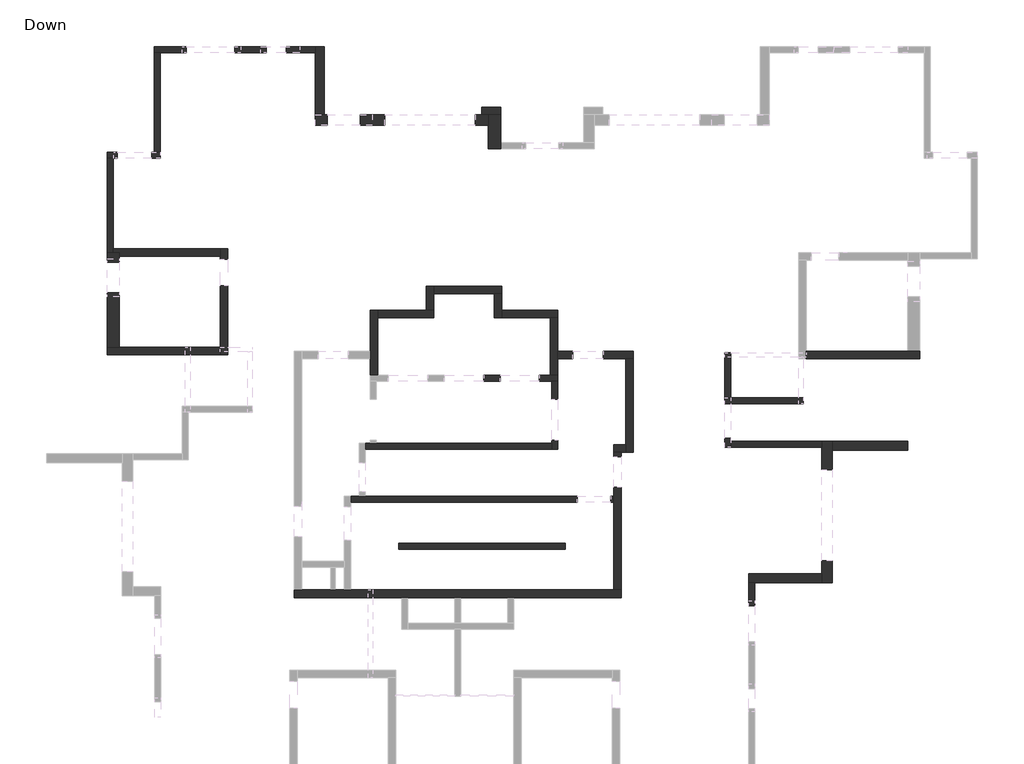
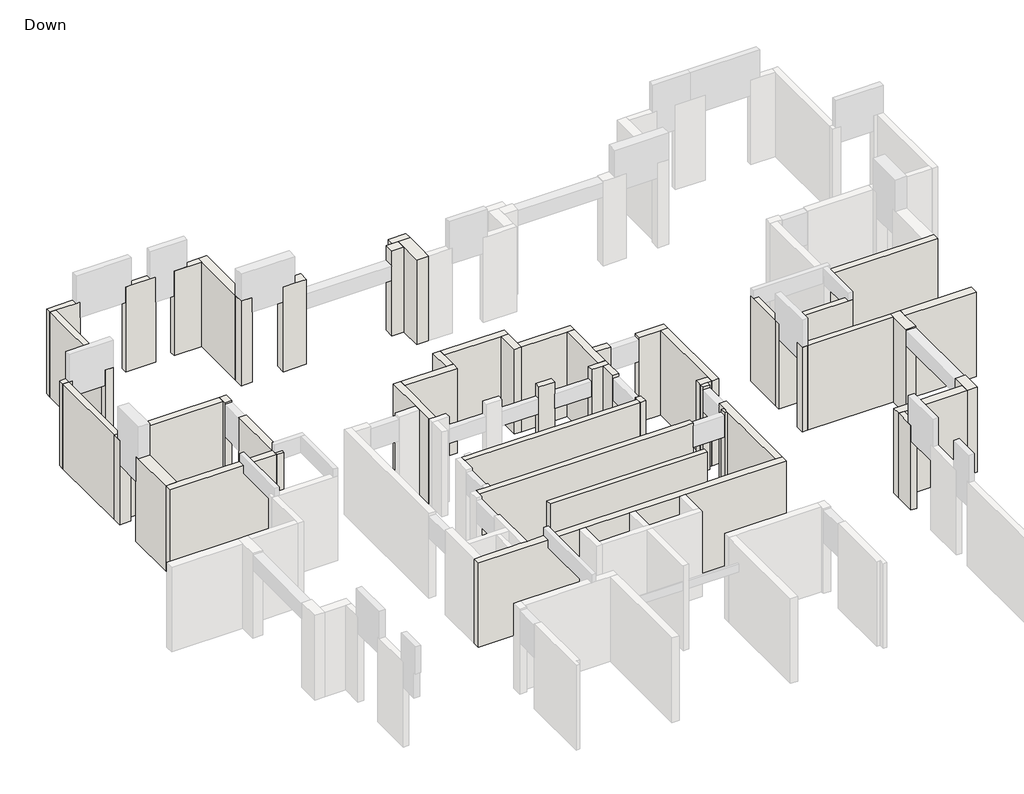
# One storey, part 2 of 3: 51 walls.
"""IFC4 building model written with IfcOpenShell, lengths in millimetres."""

from ifc_helpers import new_model, si_unit, origin, origin_with_axes, place, context, project, spatial, polyline, outline, extrude, faceted_brep, element, save

model = new_model("IFC4")

# Units and contexts
model_context = context("Model", 3, world=origin())
ifc_project = project(units=[si_unit("LENGTHUNIT", "METRE", prefix="MILLI")], contexts=[model_context])

# Site, building, storey
site = spatial("IfcSite", under=ifc_project)
building = spatial("IfcBuilding", under=site)
storey = spatial("IfcBuildingStorey", under=building, Name="Down", Elevation=0.0)

# Walls
placement = place(None, origin())
element("IfcWall", 1, ObjectType="20", at=placement, inside=storey, context=model_context, shape_type="Brep", body=[
    faceted_brep([(-24284.8686951, 10125.9195024, 0.0), (-25346.2068588, 10125.9195024, 0.0), (-25346.2068588, 10125.9195024, 3150.0), (-24424.8686951, 10125.9195024, 3150.0), (-24284.8686951, 10125.9195024, 3150.0), (-24284.8686951, 10125.9195024, 2570.0), (-24284.8686951, 9925.9195024, 0.0), (-24284.8686951, 9925.9195024, 2570.0), (-24284.8686951, 9925.9195024, 3150.0), (-24424.8686951, 9925.9195024, 3150.0), (-25146.2068588, 9925.9195024, 3150.0), (-25346.2068588, 9925.9195024, 3150.0), (-25346.2068588, 9925.9195024, 0.0), (-25146.2068588, 9925.9195024, 0.0)], [[[0, 1, 2, 3, 4, 5]], [[6, 7, 8, 9, 10, 11, 12, 13]], [[1, 0, 6, 13, 12]], [[4, 3, 2, 11, 10, 9, 8]], [[0, 5, 4, 8, 7, 6]], [[2, 1, 12, 11]]]),
])
element("IfcWall", 2, ObjectType="20", at=placement, inside=storey, context=model_context, shape_type="Brep", body=[
    faceted_brep([(-25346.2068588, 9925.9195024, 0.0), (-25346.2068588, 6620.0664514, 0.0), (-25346.2068588, 6620.0664514, 3150.0), (-25346.2068588, 9925.9195024, 3150.0), (-25146.2068588, 9925.9195024, 0.0), (-25146.2068588, 9925.9195024, 2950.0), (-25146.2068588, 9925.9195024, 3150.0), (-25146.2068588, 6620.0664514, 3150.0), (-25146.2068588, 6620.0664514, 0.0)], [[[0, 1, 2, 3]], [[4, 5, 6, 7, 8]], [[1, 0, 4, 8]], [[3, 2, 7, 6]], [[0, 3, 6, 5, 4]], [[2, 1, 8, 7]]]),
])
element("IfcWall", 3, ObjectType="20", at=placement, inside=storey, context=model_context, shape_type="Brep", body=[
    faceted_brep([(-26578.3590155, 6620.0664514, 0.0), (-26909.0507397, 6620.0664514, 0.0), (-26909.0507397, 6620.0664514, 3150.0), (-26693.7048776, 6620.0664514, 3150.0), (-26578.3590155, 6620.0664514, 3150.0), (-26578.3590155, 6620.0664514, 2570.0), (-26578.3590155, 6420.0664514, 0.0), (-26578.3590155, 6420.0664514, 2570.0), (-26578.3590155, 6420.0664514, 3150.0), (-26693.7048776, 6420.0664514, 3150.0), (-26709.0507397, 6420.0664514, 3150.0), (-26909.0507397, 6420.0664514, 3150.0), (-26909.0507397, 6420.0664514, 0.0), (-26709.0507397, 6420.0664514, 0.0)], [[[0, 1, 2, 3, 4, 5]], [[6, 7, 8, 9, 10, 11, 12, 13]], [[1, 0, 6, 13, 12]], [[4, 3, 2, 11, 10, 9, 8]], [[0, 5, 4, 8, 7, 6]], [[2, 1, 12, 11]]]),
])
element("IfcWall", 4, ObjectType="20", at=placement, inside=storey, context=model_context, shape_type="Brep", body=[
    faceted_brep([(-26909.0507397, 6420.0664514, 0.0), (-26909.0507397, 3300.0930561, 0.0), (-26909.0507397, 3300.0930561, 3150.0), (-26909.0507397, 6420.0664514, 3150.0), (-26709.0507397, 6420.0664514, 0.0), (-26709.0507397, 6420.0664514, 2950.0), (-26709.0507397, 6420.0664514, 3150.0), (-26709.0507397, 3425.0930561, 3150.0), (-26709.0507397, 3300.0930561, 3150.0), (-26709.0507397, 3300.0930561, 0.0), (-26709.0507397, 3425.0930561, 0.0)], [[[0, 1, 2, 3]], [[4, 5, 6, 7, 8, 9, 10]], [[1, 0, 4, 10, 9]], [[2, 1, 9, 8]], [[3, 2, 8, 7, 6]], [[0, 3, 6, 5, 4]]]),
])
element("IfcWall", 5, ObjectType="20", at=placement, inside=storey, context=model_context, shape_type="Brep", body=[
    faceted_brep([(-3237.9389996, -2945.5397979, 0.0), (-6249.3881109, -2945.5397979, 0.0), (-6249.3881109, -2945.5397979, 3150.0), (-3237.9389996, -2945.5397979, 3150.0), (-3237.9389996, -3145.5397979, 0.0), (-3237.9389996, -3145.5397979, 2950.0), (-3237.9389996, -3145.5397979, 3150.0), (-6249.3881109, -3145.5397979, 3150.0), (-6249.3881109, -3145.5397979, 0.0)], [[[0, 1, 2, 3]], [[4, 5, 6, 7, 8]], [[1, 0, 4, 8]], [[3, 2, 7, 6]], [[0, 3, 6, 5, 4]], [[2, 1, 8, 7]]]),
])
element("IfcWall", 6, ObjectType="20", at=placement, inside=storey, context=model_context, shape_type="Brep", body=[
    faceted_brep([(-6249.3881109, -3145.5397979, 0.0), (-6249.3881109, -2945.5397979, 0.0), (-6249.3881109, -2845.5511191, 0.0), (-6249.3881109, -2845.5511191, 2570.0), (-6249.3881109, -2845.5511191, 3150.0), (-6249.3881109, -2945.5397979, 3150.0), (-6249.3881109, -3145.5397979, 3150.0), (-6449.3881109, -3145.5397979, 0.0), (-6449.3881109, -3145.5397979, 2950.0), (-6449.3881109, -3145.5397979, 3150.0), (-6449.3881109, -2845.5511191, 3150.0), (-6449.3881109, -2845.5511191, 2570.0), (-6449.3881109, -2845.5511191, 0.0)], [[[0, 1, 2, 3, 4, 5, 6]], [[7, 8, 9, 10, 11, 12]], [[2, 1, 0, 7, 12]], [[4, 3, 2, 12, 11, 10]], [[6, 5, 4, 10, 9]], [[0, 6, 9, 8, 7]]]),
])
element("IfcWall", 7, ObjectType="20", at=placement, inside=storey, context=model_context, shape_type="Brep", body=[
    faceted_brep([(-3845.4992849, -1513.3876412, 0.0), (-6249.3881109, -1513.3876412, 0.0), (-6449.3881109, -1513.3876412, 0.0), (-6449.3881109, -1513.3876412, 3150.0), (-6249.3881109, -1513.3876412, 3150.0), (-3995.4992849, -1513.3876412, 3150.0), (-3845.4992849, -1513.3876412, 3150.0), (-3845.4992849, -1513.3876412, 2850.0), (-3845.4992849, -1713.3876412, 0.0), (-3845.4992849, -1713.3876412, 3150.0), (-3995.4992849, -1713.3876412, 3150.0), (-6249.3881109, -1713.3876412, 3150.0), (-6449.3881109, -1713.3876412, 3150.0), (-6449.3881109, -1713.3876412, 2570.0), (-6449.3881109, -1713.3876412, 0.0)], [[[0, 1, 2, 3, 4, 5, 6, 7]], [[8, 9, 10, 11, 12, 13, 14]], [[2, 1, 0, 8, 14]], [[6, 5, 4, 3, 12, 11, 10, 9]], [[0, 7, 6, 9, 8]], [[3, 2, 14, 13, 12]]]),
])
element("IfcWall", 8, ObjectType="20", at=placement, inside=storey, context=model_context, shape_type="Brep", body=[
    faceted_brep([(-6249.3881109, -1513.3876412, 0.0), (-6249.3881109, -10.4554551, 0.0), (-6249.3881109, -10.4554551, 2850.0), (-6249.3881109, -10.4554551, 3150.0), (-6249.3881109, -160.4554551, 3150.0), (-6249.3881109, -1513.3876412, 3150.0), (-6249.3881109, -1513.3876412, 2700.0), (-6249.3881109, -1513.3876412, 2550.0), (-6449.3881109, -1513.3876412, 0.0), (-6449.3881109, -1513.3876412, 3150.0), (-6449.3881109, -160.4554551, 3150.0), (-6449.3881109, -10.4554551, 3150.0), (-6449.3881109, -10.4554551, 2950.0), (-6449.3881109, -10.4554551, 0.0)], [[[0, 1, 2, 3, 4, 5, 6, 7]], [[8, 9, 10, 11, 12, 13]], [[1, 0, 8, 13]], [[3, 2, 1, 13, 12, 11]], [[5, 4, 3, 11, 10, 9]], [[0, 7, 6, 5, 9, 8]]]),
])
element("IfcWall", 9, ObjectType="20", at=placement, inside=storey, context=model_context, shape_type="Brep", body=[
    faceted_brep([(-10126.055155, -4768.7708633, 0.0), (-10226.0438338, -4768.7708633, 0.0), (-10226.0438338, -4768.7708633, 2250.0), (-10226.0438338, -4768.7708633, 3050.0), (-10226.0438338, -4768.7708633, 3150.0), (-10126.055155, -4768.7708633, 3150.0), (-10126.055155, -4768.7708633, 2950.0), (-10126.055155, -4968.7708633, 0.0), (-10126.055155, -4968.7708633, 2950.0), (-10126.055155, -4968.7708633, 3150.0), (-10226.0438338, -4968.7708633, 3150.0), (-10226.0438338, -4968.7708633, 3050.0), (-10226.0438338, -4968.7708633, 2250.0), (-10226.0438338, -4968.7708633, 0.0)], [[[0, 1, 2, 3, 4, 5, 6]], [[7, 8, 9, 10, 11, 12, 13]], [[1, 0, 7, 13]], [[4, 3, 2, 1, 13, 12, 11, 10]], [[5, 4, 10, 9]], [[0, 6, 5, 9, 8, 7]]]),
])
element("IfcWall", 10, ObjectType="20", at=placement, inside=storey, context=model_context, shape_type="Brep", body=[
    faceted_brep([(-11328.0023982, -4768.7708633, 0.0), (-18350.1013454, -4768.7708633, 0.0), (-18550.1013454, -4768.7708633, 0.0), (-18843.2746727, -4768.7708633, 0.0), (-18843.2746727, -4768.7708633, 3150.0), (-18550.1013454, -4768.7708633, 3150.0), (-18350.1013454, -4768.7708633, 3150.0), (-16646.6710273, -4768.7708633, 3150.0), (-14282.8761671, -4768.7708633, 3150.0), (-11328.0023982, -4768.7708633, 3150.0), (-11328.0023982, -4768.7708633, 3050.0), (-11328.0023982, -4768.7708633, 2250.0), (-11328.0023982, -4968.7708633, 0.0), (-11328.0023982, -4968.7708633, 2250.0), (-11328.0023982, -4968.7708633, 3050.0), (-11328.0023982, -4968.7708633, 3150.0), (-11723.2701442, -4968.7708633, 3150.0), (-17252.8523926, -4968.7708633, 3150.0), (-18843.2746727, -4968.7708633, 3150.0), (-18843.2746727, -4968.7708633, 2950.0), (-18843.2746727, -4968.7708633, 0.0)], [[[0, 1, 2, 3, 4, 5, 6, 7, 8, 9, 10, 11]], [[12, 13, 14, 15, 16, 17, 18, 19, 20]], [[3, 2, 1, 0, 12, 20]], [[9, 8, 7, 6, 5, 4, 18, 17, 16, 15]], [[0, 11, 10, 9, 15, 14, 13, 12]], [[4, 3, 20, 19, 18]]]),
])
element("IfcWall", 11, ObjectType="20", at=placement, inside=storey, context=model_context, shape_type="Brep", body=[
    faceted_brep([(-11984.1523396, -762.4325886, 0.0), (-12234.1523396, -762.4325886, 0.0), (-12584.1498, -762.4325886, 0.0), (-12584.1498, -762.4325886, 3150.0), (-12234.1523396, -762.4325886, 3150.0), (-11984.1523396, -762.4325886, 3150.0), (-11984.1498, -962.4325886, 0.0), (-11984.1498, -962.4325886, 3150.0), (-12184.178103, -962.4325886, 3150.0), (-12584.1498, -962.4325886, 3150.0), (-12584.1498, -962.4325886, 0.0), (-12184.178103, -962.4325886, 0.0)], [[[0, 1, 2, 3, 4, 5]], [[6, 7, 8, 9, 10, 11]], [[2, 1, 0, 6, 11, 10]], [[3, 2, 10, 9]], [[5, 4, 3, 9, 8, 7]], [[0, 5, 7, 6]]]),
])
element("IfcWall", 12, ObjectType="20", at=placement, inside=storey, context=model_context, shape_type="Brep", body=[
    faceted_brep([(-13887.0876467, -762.4310014, 0.0), (-14438.066929, -762.4310014, 0.0), (-14438.066929, -762.4310014, 2150.0), (-14438.066929, -762.4310014, 2700.0), (-14438.066929, -762.4310014, 3150.0), (-13887.0876467, -762.4310014, 3150.0), (-13887.0876467, -762.4310014, 2700.0), (-13887.0876467, -762.4310014, 2150.0), (-13887.0876467, -962.4310014, 0.0), (-13887.0876467, -962.4310014, 2150.0), (-13887.0876467, -962.4310014, 2700.0), (-13887.0876467, -962.4310014, 3150.0), (-14438.066929, -962.4310014, 3150.0), (-14438.066929, -962.4310014, 2700.0), (-14438.066929, -962.4310014, 2150.0), (-14438.066929, -962.4310014, 0.0)], [[[0, 1, 2, 3, 4, 5, 6, 7]], [[8, 9, 10, 11, 12, 13, 14, 15]], [[1, 0, 8, 15]], [[4, 3, 2, 1, 15, 14, 13, 12]], [[5, 4, 12, 11]], [[0, 7, 6, 5, 11, 10, 9, 8]]]),
])
element("IfcWall", 13, ObjectType="20", at=placement, inside=storey, context=model_context, shape_type="Brep", body=[
    faceted_brep([(-11984.178103, -1563.404623, 0.0), (-11984.178103, -962.4325886, 0.0), (-11984.178103, -962.4325886, 3150.0), (-11984.178103, -1563.404623, 3150.0), (-11984.178103, -1563.404623, 3050.0), (-11984.178103, -1563.404623, 2250.0), (-12184.178103, -1563.404623, 0.0), (-12184.178103, -1563.404623, 2250.0), (-12184.178103, -1563.404623, 3050.0), (-12184.178103, -1563.404623, 3150.0), (-12184.178103, -962.4325886, 3150.0), (-12184.178103, -962.4325886, 2950.0), (-12184.178103, -962.4325886, 0.0)], [[[0, 1, 2, 3, 4, 5]], [[6, 7, 8, 9, 10, 11, 12]], [[1, 0, 6, 12]], [[3, 2, 10, 9]], [[0, 5, 4, 3, 9, 8, 7, 6]], [[2, 1, 12, 11, 10]]]),
])
element("IfcWall", 14, ObjectType="20", at=placement, inside=storey, context=model_context, shape_type="Brep", body=[
    faceted_brep([(-12184.178103, -2915.3348845, 0.0), (-12184.178103, -3015.8216954, 0.0), (-12184.178103, -3215.8216954, 0.0), (-12184.178103, -3215.8216954, 3150.0), (-12184.178103, -3015.8216954, 3150.0), (-12184.178103, -2915.3348845, 3150.0), (-12184.178103, -2915.3348845, 3050.0), (-12184.178103, -2915.3348845, 2250.0), (-11984.178103, -2915.3348845, 0.0), (-11984.178103, -2915.3348845, 2250.0), (-11984.178103, -2915.3348845, 3050.0), (-11984.178103, -2915.3348845, 3150.0), (-11984.178103, -3215.8216954, 3150.0), (-11984.178103, -3215.8216954, 2950.0), (-11984.178103, -3215.8216954, 0.0)], [[[0, 1, 2, 3, 4, 5, 6, 7]], [[8, 9, 10, 11, 12, 13, 14]], [[2, 1, 0, 8, 14]], [[5, 4, 3, 12, 11]], [[0, 7, 6, 5, 11, 10, 9, 8]], [[3, 2, 14, 13, 12]]]),
])
element("IfcWall", 15, ObjectType="20", at=placement, inside=storey, context=model_context, shape_type="Brep", body=[
    faceted_brep([(-12184.178103, -3015.8216954, 0.0), (-17993.9143195, -3015.8216954, 0.0), (-18193.9143195, -3015.8216954, 0.0), (-18350.1013454, -3015.8216954, 0.0), (-18350.1013454, -3015.8216954, 3150.0), (-18193.9143195, -3015.8216954, 3150.0), (-17993.9143195, -3015.8216954, 3150.0), (-12184.178103, -3015.8216954, 3150.0), (-12184.178103, -3015.8216954, 2950.0), (-12184.178103, -3215.8216954, 0.0), (-12184.178103, -3215.8216954, 3150.0), (-14282.8761671, -3215.8216954, 3150.0), (-16646.6710273, -3215.8216954, 3150.0), (-18350.1013454, -3215.8216954, 3150.0), (-18350.1013454, -3215.8216954, 2950.0), (-18350.1013454, -3215.8216954, 0.0)], [[[0, 1, 2, 3, 4, 5, 6, 7, 8]], [[9, 10, 11, 12, 13, 14, 15]], [[3, 2, 1, 0, 9, 15]], [[7, 6, 5, 4, 13, 12, 11, 10]], [[0, 8, 7, 10, 9]], [[4, 3, 15, 14, 13]]]),
])
element("IfcWall", 16, ObjectType="20", at=placement, inside=storey, context=model_context, shape_type="Brep", body=[
    faceted_brep([(-25146.2068588, 6620.0664514, 0.0), (-25346.2068588, 6620.0664514, 0.0), (-25426.4061116, 6620.0664514, 0.0), (-25426.4061116, 6620.0664514, 2570.0), (-25426.4061116, 6620.0664514, 3150.0), (-25346.2068588, 6620.0664514, 3150.0), (-25146.2068588, 6620.0664514, 3150.0), (-25146.2068588, 6420.0664514, 0.0), (-25146.2068588, 6420.0664514, 2950.0), (-25146.2068588, 6420.0664514, 3150.0), (-25426.4061116, 6420.0664514, 3150.0), (-25426.4061116, 6420.0664514, 2570.0), (-25426.4061116, 6420.0664514, 0.0)], [[[0, 1, 2, 3, 4, 5, 6]], [[7, 8, 9, 10, 11, 12]], [[2, 1, 0, 7, 12]], [[4, 3, 2, 12, 11, 10]], [[6, 5, 4, 10, 9]], [[0, 6, 9, 8, 7]]]),
])
element("IfcWall", 17, ObjectType="20", at=placement, inside=storey, context=model_context, shape_type="Brep", body=[
    faceted_brep([(-22681.9251878, 9925.9195024, 0.0), (-21629.9609627, 9925.9195024, 0.0), (-21629.9609627, 9925.9195024, 3150.0), (-22484.8686951, 9925.9195024, 3150.0), (-22681.9251878, 9925.9195024, 3150.0), (-22681.9251878, 9925.9195024, 2570.0), (-22681.9251878, 10125.9195024, 0.0), (-22681.9251878, 10125.9195024, 2570.0), (-22681.9251878, 10125.9195024, 3150.0), (-22484.8686951, 10125.9195024, 3150.0), (-21809.9609627, 10125.9195024, 3150.0), (-21629.9609627, 10125.9195024, 3150.0), (-21629.9609627, 10125.9195024, 2220.0), (-21629.9609627, 10125.9195024, 0.0), (-21629.9609627, 9926.4176344, 3150.0)], [[[0, 1, 2, 3, 4, 5]], [[6, 7, 8, 9, 10, 11, 12, 13]], [[1, 0, 6, 13]], [[2, 1, 13, 12, 11, 14]], [[4, 3, 2, 14, 11, 10, 9, 8]], [[0, 5, 4, 8, 7, 6]]]),
])
element("IfcWall", 18, ObjectType="20", at=placement, inside=storey, context=model_context, shape_type="Brep", body=[
    faceted_brep([(-20978.9930017, 9925.9195024, 0.0), (-20006.7412186, 9925.9195024, 0.0), (-20006.7412186, 9925.9195024, 2950.0), (-20006.7412186, 9925.9195024, 3150.0), (-20978.9930017, 9925.9195024, 3150.0), (-20978.9930017, 10125.9195024, 0.0), (-20978.9930017, 10125.9195024, 2220.0), (-20978.9930017, 10125.9195024, 3150.0), (-20529.9609627, 10125.9195024, 3150.0), (-20006.7412186, 10125.9195024, 3150.0), (-20006.7412186, 10125.9195024, 0.0), (-20978.9930017, 9926.4176344, 3150.0)], [[[0, 1, 2, 3, 4]], [[5, 6, 7, 8, 9, 10]], [[1, 0, 5, 10]], [[4, 3, 9, 8, 7, 11]], [[0, 4, 11, 7, 6, 5]], [[3, 2, 1, 10, 9]]]),
])
element("IfcWall", 19, ObjectType="20", at=placement, inside=storey, context=model_context, shape_type="Brep", body=[
    faceted_brep([(-5448.4371316, -8389.7150498, 0.0), (-5448.4371316, -7643.0129016, 0.0), (-5448.4371316, -7643.0129016, 3150.0), (-5448.4371316, -8231.6622931, 3150.0), (-5448.4371316, -8389.7150498, 3150.0), (-5448.4371316, -8389.7150498, 2570.0), (-5648.4371316, -8389.7150498, 0.0), (-5648.4371316, -8389.7150498, 2570.0), (-5648.4371316, -8389.7150498, 3150.0), (-5648.4371316, -8231.6622931, 3150.0), (-5648.4371316, -7643.0129016, 3150.0), (-5648.4371316, -7643.0129016, 0.0)], [[[0, 1, 2, 3, 4, 5]], [[6, 7, 8, 9, 10, 11]], [[1, 0, 6, 11]], [[4, 3, 2, 10, 9, 8]], [[0, 5, 4, 8, 7, 6]], [[2, 1, 11, 10]]]),
])
element("IfcWall", 20, ObjectType="20", at=placement, inside=storey, context=model_context, shape_type="SweptSolid", body=[
    extrude(outline(polyline([(-11723.2701442, -6521.6973888), (-17252.8523926, -6521.6973888), (-17252.8523926, -6321.6973888), (-11723.2701442, -6321.6973888), (-11723.2701442, -6521.6973888)])), origin_with_axes(), (0.0, 0.0, 1.0), 3150.0),
])
element("IfcWall", 21, ObjectType="25", at=placement, inside=storey, context=model_context, shape_type="Brep", body=[
    faceted_brep([(-26509.0507397, 3175.0930561, 0.0), (-23152.2127458, 3175.0930561, 0.0), (-23152.2127458, 3175.0930561, 2860.0), (-23152.2127458, 3175.0930561, 3150.0), (-26509.0507397, 3175.0930561, 3150.0), (-26509.0507397, 3175.0930561, 2860.0), (-26709.0507397, 3425.0930561, 0.0), (-26709.0507397, 3425.0930561, 2950.0), (-26709.0507397, 3425.0930561, 3150.0), (-23152.2127458, 3425.0930561, 3150.0), (-23152.2127458, 3425.0930561, 0.0), (-26509.0507397, 3300.0930561, 0.0), (-26709.0507397, 3300.0930561, 0.0), (-26709.0507397, 3300.0930561, 3150.0), (-26509.0507397, 3300.0930561, 3150.0)], [[[0, 1, 2, 3, 4, 5]], [[6, 7, 8, 9, 10]], [[1, 0, 11, 12, 6, 10]], [[4, 3, 9, 8, 13, 14]], [[3, 2, 1, 10, 9]], [[0, 5, 4, 14, 11]], [[14, 13, 12, 11]], [[13, 8, 7, 6, 12]]]),
])
element("IfcWall", 22, ObjectType="25", at=placement, inside=storey, context=model_context, shape_type="Brep", body=[
    faceted_brep([(-23152.2127458, 3425.0930561, 0.0), (-23152.2127458, 3175.0930561, 0.0), (-23152.2127458, 3085.0930561, 0.0), (-23152.2127458, 3085.0930561, 1900.0), (-23152.2127458, 3085.0930561, 3100.0), (-23152.2127458, 3085.0930561, 3150.0), (-23152.2127458, 3175.0930561, 3150.0), (-23152.2127458, 3425.0930561, 3150.0), (-22902.2127458, 3425.0930561, 0.0), (-22902.2127458, 3425.0930561, 2950.0), (-22902.2127458, 3425.0930561, 3150.0), (-22902.2127458, 3085.0930561, 3150.0), (-22902.2127458, 3085.0930561, 3100.0), (-22902.2127458, 3085.0930561, 1900.0), (-22902.2127458, 3085.0930561, 0.0)], [[[0, 1, 2, 3, 4, 5, 6, 7]], [[8, 9, 10, 11, 12, 13, 14]], [[2, 1, 0, 8, 14]], [[5, 4, 3, 2, 14, 13, 12, 11]], [[7, 6, 5, 11, 10]], [[0, 7, 10, 9, 8]]]),
])
element("IfcWall", 23, ObjectType="25", at=placement, inside=storey, context=model_context, shape_type="Brep", body=[
    faceted_brep([(-23152.2127458, 2208.0433561, 0.0), (-23152.2127458, 170.2815538, 0.0), (-23152.2127458, -79.7184462, 0.0), (-23152.2127458, -79.7184462, 3150.0), (-23152.2127458, 20.2815538, 3150.0), (-23152.2127458, 170.2815538, 3150.0), (-23152.2127458, 2208.0433561, 3150.0), (-23152.2127458, 2208.0433561, 3100.0), (-23152.2127458, 2208.0433561, 1900.0), (-22902.2127458, 2208.0433561, 0.0), (-22902.2127458, 2208.0433561, 1900.0), (-22902.2127458, 2208.0433561, 3100.0), (-22902.2127458, 2208.0433561, 3150.0), (-22902.2127458, 170.2815538, 3150.0), (-22902.2127458, 20.2815538, 3150.0), (-22902.2127458, -79.7184462, 3150.0), (-22902.2127458, -79.7184462, 2700.0), (-22902.2127458, -79.7184462, 2550.0), (-22902.2127458, -79.7184462, 0.0)], [[[0, 1, 2, 3, 4, 5, 6, 7, 8]], [[9, 10, 11, 12, 13, 14, 15, 16, 17, 18]], [[2, 1, 0, 9, 18]], [[6, 5, 4, 3, 15, 14, 13, 12]], [[0, 8, 7, 6, 12, 11, 10, 9]], [[3, 2, 18, 17, 16, 15]]]),
])
element("IfcWall", 24, ObjectType="25", at=placement, inside=storey, context=model_context, shape_type="Brep", body=[
    faceted_brep([(-23152.2127458, 170.2815538, 0.0), (-26509.0507397, 170.2815538, 0.0), (-26909.0507397, 170.2815538, 0.0), (-26909.0507397, 170.2815538, 3150.0), (-26509.0507397, 170.2815538, 3150.0), (-24310.0622873, 170.2815538, 3150.0), (-24160.0622873, 170.2815538, 3150.0), (-23152.2127458, 170.2815538, 3150.0), (-23152.2127458, 170.2815538, 2860.0), (-23152.2127458, -79.7184462, 0.0), (-23152.2127458, -79.7184462, 3150.0), (-24160.0622873, -79.7184462, 3150.0), (-24310.0622873, -79.7184462, 3150.0), (-26909.0507397, -79.7184462, 3150.0), (-26909.0507397, -79.7184462, 0.0)], [[[0, 1, 2, 3, 4, 5, 6, 7, 8]], [[9, 10, 11, 12, 13, 14]], [[2, 1, 0, 9, 14]], [[7, 6, 5, 4, 3, 13, 12, 11, 10]], [[0, 8, 7, 10, 9]], [[3, 2, 14, 13]]]),
])
element("IfcWall", 25, ObjectType="25", at=placement, inside=storey, context=model_context, shape_type="Brep", body=[
    faceted_brep([(-3745.4992849, -210.9535871, 0.0), (11.338709, -210.9535871, 0.0), (11.338709, -210.9535871, 3150.0), (-3745.4992849, -210.9535871, 3150.0), (-3745.4992849, 39.0464129, 0.0), (-3745.4992849, 39.0464129, 2860.0), (-3745.4992849, 39.0464129, 3150.0), (-388.661291, 39.0464129, 3150.0), (11.338709, 39.0464129, 3150.0), (11.338709, 39.0464129, 0.0), (-388.661291, 39.0464129, 0.0)], [[[0, 1, 2, 3]], [[4, 5, 6, 7, 8, 9, 10]], [[1, 0, 4, 10, 9]], [[3, 2, 8, 7, 6]], [[0, 3, 6, 5, 4]], [[2, 1, 9, 8]]]),
])
element("IfcWall", 26, ObjectType="25", at=placement, inside=storey, context=model_context, shape_type="Brep", body=[
    faceted_brep([(-20703.5033605, -8124.1201217, 0.0), (-17147.6559701, -8124.1201217, 0.0), (-16947.6559701, -8124.1201217, 0.0), (-15389.5443432, -8124.1201217, 0.0), (-15189.5443432, -8124.1201217, 0.0), (-13631.410074, -8124.1201217, 0.0), (-13431.410074, -8124.1201217, 0.0), (-9876.055155, -8124.1201217, 0.0), (-9876.055155, -8124.1201217, 2950.0), (-9876.055155, -8124.1201217, 3150.0), (-12485.911942, -8124.1201217, 3150.0), (-12635.911942, -8124.1201217, 3150.0), (-13431.410074, -8124.1201217, 3150.0), (-13631.410074, -8124.1201217, 3150.0), (-15189.5443432, -8124.1201217, 3150.0), (-15389.5443432, -8124.1201217, 3150.0), (-16947.6559701, -8124.1201217, 3150.0), (-17147.6559701, -8124.1201217, 3150.0), (-18103.1541021, -8124.1201217, 3150.0), (-18253.1541021, -8124.1201217, 3150.0), (-20703.5033605, -8124.1201217, 3150.0), (-20703.5033605, -8124.1201217, 2950.0), (-20703.5033605, -7874.1201217, 0.0), (-20703.5033605, -7874.1201217, 2950.0), (-20703.5033605, -7874.1201217, 3150.0), (-20703.0108891, -7874.1201217, 3150.0), (-20453.0108891, -7874.1201217, 3150.0), (-19501.573099, -7874.1201217, 3150.0), (-19351.573099, -7874.1201217, 3150.0), (-19043.2746727, -7874.1201217, 3150.0), (-18843.2746727, -7874.1201217, 3150.0), (-18253.1541021, -7874.1201217, 3150.0), (-18103.1541021, -7874.1201217, 3150.0), (-17252.8523926, -7874.1201217, 3150.0), (-12635.911942, -7874.1201217, 3150.0), (-12485.911942, -7874.1201217, 3150.0), (-11723.2701442, -7874.1201217, 3150.0), (-10126.055155, -7874.1201217, 3150.0), (-9876.055155, -7874.1201217, 3150.0), (-9876.055155, -7874.1201217, 0.0), (-10126.055155, -7874.1201217, 0.0), (-18843.2746727, -7874.1201217, 0.0), (-19043.2746727, -7874.1201217, 0.0), (-19351.573099, -7874.1201217, 0.0), (-19501.573099, -7874.1201217, 0.0), (-20453.0108891, -7874.1201217, 0.0), (-20703.0108891, -7874.1201217, 0.0)], [[[0, 1, 2, 3, 4, 5, 6, 7, 8, 9, 10, 11, 12, 13, 14, 15, 16, 17, 18, 19, 20, 21]], [[22, 23, 24, 25, 26, 27, 28, 29, 30, 31, 32, 33, 34, 35, 36, 37, 38, 39, 40, 41, 42, 43, 44, 45, 46]], [[7, 6, 5, 4, 3, 2, 1, 0, 22, 46, 45, 44, 43, 42, 41, 40, 39]], [[20, 19, 18, 17, 16, 15, 14, 13, 12, 11, 10, 9, 38, 37, 36, 35, 34, 33, 32, 31, 30, 29, 28, 27, 26, 25, 24]], [[0, 21, 20, 24, 23, 22]], [[9, 8, 7, 39, 38]]]),
])
element("IfcWall", 27, ObjectType="25", at=placement, inside=storey, context=model_context, shape_type="Brep", body=[
    faceted_brep([(-9876.055155, -7874.1201217, 0.0), (-9876.055155, -4468.2840524, 0.0), (-9876.055155, -4468.2840524, 2250.0), (-9876.055155, -4468.2840524, 3050.0), (-9876.055155, -4468.2840524, 3150.0), (-9876.055155, -7874.1201217, 3150.0), (-10126.055155, -7874.1201217, 0.0), (-10126.055155, -7874.1201217, 2950.0), (-10126.055155, -7874.1201217, 3150.0), (-10126.055155, -4968.7708633, 3150.0), (-10126.055155, -4768.7708633, 3150.0), (-10126.055155, -4468.2840524, 3150.0), (-10126.055155, -4468.2840524, 3050.0), (-10126.055155, -4468.2840524, 2250.0), (-10126.055155, -4468.2840524, 0.0), (-10126.055155, -4768.7708633, 0.0), (-10126.055155, -4968.7708633, 0.0)], [[[0, 1, 2, 3, 4, 5]], [[6, 7, 8, 9, 10, 11, 12, 13, 14, 15, 16]], [[1, 0, 6, 16, 15, 14]], [[4, 3, 2, 1, 14, 13, 12, 11]], [[5, 4, 11, 10, 9, 8]], [[0, 5, 8, 7, 6]]]),
])
element("IfcWall", 28, ObjectType="25", at=placement, inside=storey, context=model_context, shape_type="Brep", body=[
    faceted_brep([(-18194.4124515, 1391.4691458, 0.0), (-18194.4124515, 39.5388843, 0.0), (-18194.4124515, -210.4611157, 0.0), (-18194.4124515, -762.4310014, 0.0), (-18194.4124515, -762.4310014, 3150.0), (-18194.4124515, -210.4611157, 3150.0), (-18194.4124515, 39.5388843, 3150.0), (-18194.4124515, 1391.4691458, 3150.0), (-18194.4124515, 1391.4691458, 2950.0), (-17944.4124515, 1391.4691458, 0.0), (-17944.4124515, 1391.4691458, 3150.0), (-17944.4124515, 1141.4691458, 3150.0), (-17944.4124515, -762.4310014, 3150.0), (-17944.4124515, -762.4310014, 0.0), (-17944.4124515, 1141.4691458, 0.0)], [[[0, 1, 2, 3, 4, 5, 6, 7, 8]], [[9, 10, 11, 12, 13, 14]], [[3, 2, 1, 0, 9, 14, 13]], [[7, 6, 5, 4, 12, 11, 10]], [[0, 8, 7, 10, 9]], [[4, 3, 13, 12]]]),
])
element("IfcWall", 29, ObjectType="25", at=placement, inside=storey, context=model_context, shape_type="Brep", body=[
    faceted_brep([(-17944.4124515, 1141.4691458, 0.0), (-16091.0047757, 1141.4691458, 0.0), (-16091.0047757, 1141.4691458, 3150.0), (-17944.4124515, 1141.4691458, 3150.0), (-17944.4124515, 1391.4691458, 0.0), (-17944.4124515, 1391.4691458, 3150.0), (-16341.0047757, 1391.4691458, 3150.0), (-16091.0047757, 1391.4691458, 3150.0), (-16091.0047757, 1391.4691458, 0.0), (-16341.0047757, 1391.4691458, 0.0)], [[[0, 1, 2, 3]], [[4, 5, 6, 7, 8, 9]], [[1, 0, 4, 9, 8]], [[3, 2, 7, 6, 5]], [[0, 3, 5, 4]], [[2, 1, 8, 7]]]),
])
element("IfcWall", 30, ObjectType="25", at=placement, inside=storey, context=model_context, shape_type="Brep", body=[
    faceted_brep([(-16091.0047757, 1391.4691458, 0.0), (-16091.0047757, 1942.9408995, 0.0), (-16091.0047757, 2192.9408995, 0.0), (-16091.0047757, 2192.9408995, 3150.0), (-16091.0047757, 1942.9408995, 3150.0), (-16091.0047757, 1391.4691458, 3150.0), (-16341.0047757, 1391.4691458, 0.0), (-16341.0047757, 1391.4691458, 2950.0), (-16341.0047757, 1391.4691458, 3150.0), (-16341.0047757, 2192.9408995, 3150.0), (-16341.0047757, 2192.9408995, 2950.0), (-16341.0047757, 2192.9408995, 0.0)], [[[0, 1, 2, 3, 4, 5]], [[6, 7, 8, 9, 10, 11]], [[2, 1, 0, 6, 11]], [[5, 4, 3, 9, 8]], [[0, 5, 8, 7, 6]], [[3, 2, 11, 10, 9]]]),
])
element("IfcWall", 31, ObjectType="25", at=placement, inside=storey, context=model_context, shape_type="Brep", body=[
    faceted_brep([(-16091.0047757, 1942.9408995, 0.0), (-14087.0933073, 1942.9408995, 0.0), (-13837.0933073, 1942.9408995, 0.0), (-13837.0933073, 1942.9408995, 3150.0), (-14087.0933073, 1942.9408995, 3150.0), (-16091.0047757, 1942.9408995, 3150.0), (-16091.0047757, 2192.9408995, 0.0), (-16091.0047757, 2192.9408995, 3150.0), (-13837.0933073, 2192.9408995, 3150.0), (-13837.0933073, 2192.9408995, 2950.0), (-13837.0933073, 2192.9408995, 0.0)], [[[0, 1, 2, 3, 4, 5]], [[6, 7, 8, 9, 10]], [[2, 1, 0, 6, 10]], [[5, 4, 3, 8, 7]], [[0, 5, 7, 6]], [[3, 2, 10, 9, 8]]]),
])
element("IfcWall", 32, ObjectType="25", at=placement, inside=storey, context=model_context, shape_type="Brep", body=[
    faceted_brep([(-14087.0933073, 1942.9408995, 0.0), (-14087.0933073, 1141.4974488, 0.0), (-14087.0933073, 1141.4974488, 3150.0), (-14087.0933073, 1942.9408995, 3150.0), (-13837.0933073, 1942.9408995, 0.0), (-13837.0933073, 1942.9408995, 3150.0), (-13837.0933073, 1391.4974488, 3150.0), (-13837.0933073, 1141.4974488, 3150.0), (-13837.0933073, 1141.4974488, 0.0), (-13837.0933073, 1391.4974488, 0.0)], [[[0, 1, 2, 3]], [[4, 5, 6, 7, 8, 9]], [[1, 0, 4, 9, 8]], [[3, 2, 7, 6, 5]], [[0, 3, 5, 4]], [[2, 1, 8, 7]]]),
])
element("IfcWall", 33, ObjectType="25", at=placement, inside=storey, context=model_context, shape_type="Brep", body=[
    faceted_brep([(-13837.0933073, 1141.4974488, 0.0), (-12234.1765157, 1141.4974488, 0.0), (-11984.1765157, 1141.4974488, 0.0), (-11984.1765157, 1141.4974488, 3150.0), (-12234.1765157, 1141.4974488, 3150.0), (-13837.0933073, 1141.4974488, 3150.0), (-13837.0933073, 1391.4974488, 0.0), (-13837.0933073, 1391.4974488, 2950.0), (-13837.0933073, 1391.4974488, 3150.0), (-11984.1796902, 1391.4974488, 3150.0), (-11984.1796902, 1391.4974488, 2950.0), (-11984.1796902, 1391.4974488, 0.0)], [[[0, 1, 2, 3, 4, 5]], [[6, 7, 8, 9, 10, 11]], [[2, 1, 0, 6, 11]], [[5, 4, 3, 9, 8]], [[0, 5, 8, 7, 6]], [[3, 2, 11, 10, 9]]]),
])
element("IfcWall", 34, ObjectType="25", at=placement, inside=storey, context=model_context, shape_type="Brep", body=[
    faceted_brep([(-12234.1765157, 1141.4974488, 0.0), (-12234.1523396, -762.4325886, 0.0), (-12234.1523396, -762.4325886, 3150.0), (-12234.1765157, 1141.4974488, 3150.0), (-11984.1765157, 1141.4974488, 0.0), (-11984.1765157, 1141.4974488, 3150.0), (-11984.1625168, 39.0464129, 3150.0), (-11984.1593423, -210.9535869, 3150.0), (-11984.1523396, -762.4325886, 3150.0), (-11984.1523396, -762.4325886, 0.0), (-11984.1593423, -210.9535871, 0.0), (-11984.1625168, 39.0464129, 0.0)], [[[0, 1, 2, 3]], [[4, 5, 6, 7, 8, 9, 10, 11]], [[1, 0, 4, 11, 10, 9]], [[3, 2, 8, 7, 6, 5]], [[0, 3, 5, 4]], [[2, 1, 9, 8]]]),
])
element("IfcWall", 35, ObjectType="25", at=placement, inside=storey, context=model_context, shape_type="Brep", body=[
    faceted_brep([(-11984.1593423, -210.9535871, 0.0), (-11477.9854165, -210.9535871, 0.0), (-11477.9854165, -210.9535871, 2250.0), (-11477.9854165, -210.9535871, 3050.0), (-11477.9854165, -210.9535871, 3150.0), (-11984.1593423, -210.9535871, 3150.0), (-11984.1625168, 39.0464129, 0.0), (-11984.1625168, 39.0464129, 2950.0), (-11984.1625168, 39.0464129, 3150.0), (-11477.9854165, 39.0464129, 3150.0), (-11477.9854165, 39.0464129, 3050.0), (-11477.9854165, 39.0464129, 2250.0), (-11477.9854165, 39.0464129, 0.0)], [[[0, 1, 2, 3, 4, 5]], [[6, 7, 8, 9, 10, 11, 12]], [[1, 0, 6, 12]], [[4, 3, 2, 1, 12, 11, 10, 9]], [[5, 4, 9, 8]], [[0, 5, 8, 7, 6]]]),
])
element("IfcWall", 36, ObjectType="25", at=placement, inside=storey, context=model_context, shape_type="Brep", body=[
    faceted_brep([(-10476.5363052, -210.9535871, 0.0), (-9724.5664195, -210.9535871, 0.0), (-9474.5664195, -210.9535871, 0.0), (-9474.5664195, -210.9535871, 3150.0), (-9724.5664195, -210.9535871, 3150.0), (-10476.5363052, -210.9535871, 3150.0), (-10476.5363052, -210.9535871, 3050.0), (-10476.5363052, -210.9535871, 2250.0), (-10476.5363052, 39.0464129, 0.0), (-10476.5363052, 39.0464129, 2250.0), (-10476.5363052, 39.0464129, 3050.0), (-10476.5363052, 39.0464129, 3150.0), (-9474.5664195, 39.0464129, 3150.0), (-9474.5664195, 39.0464129, 2950.0), (-9474.5664195, 39.0464129, 0.0), (-9474.5664195, -10.4554551, 3150.0)], [[[0, 1, 2, 3, 4, 5, 6, 7]], [[8, 9, 10, 11, 12, 13, 14]], [[2, 1, 0, 8, 14]], [[5, 4, 3, 15, 12, 11]], [[0, 7, 6, 5, 11, 10, 9, 8]], [[3, 2, 14, 13, 12, 15]]]),
])
element("IfcWall", 37, ObjectType="25", at=placement, inside=storey, context=model_context, shape_type="Brep", body=[
    faceted_brep([(-9724.5664195, -210.9535871, 0.0), (-9724.5664195, -3066.3311485, 0.0), (-9724.5664195, -3316.3311485, 0.0), (-9724.5664195, -3316.3311485, 3150.0), (-9724.5664195, -3066.3311485, 3150.0), (-9724.5664195, -210.9535871, 3150.0), (-9724.5664195, -210.9535871, 2950.0), (-9474.5664195, -210.9535871, 0.0), (-9474.5664195, -210.9535871, 3150.0), (-9474.5664195, -3316.3311485, 3150.0), (-9474.5664195, -3316.3311485, 2950.0), (-9474.5664195, -3316.3311485, 0.0)], [[[0, 1, 2, 3, 4, 5, 6]], [[7, 8, 9, 10, 11]], [[2, 1, 0, 7, 11]], [[5, 4, 3, 9, 8]], [[0, 6, 5, 8, 7]], [[3, 2, 11, 10, 9]]]),
])
element("IfcWall", 38, ObjectType="25", at=placement, inside=storey, context=model_context, shape_type="Brep", body=[
    faceted_brep([(-9724.5664195, -3066.3311485, 0.0), (-10126.055155, -3066.3311485, 0.0), (-10126.055155, -3066.3311485, 2950.0), (-10126.055155, -3066.3311485, 3150.0), (-9724.5664195, -3066.3311485, 3150.0), (-9724.5664195, -3066.3311485, 2950.0), (-9724.5664195, -3316.3311485, 0.0), (-9724.5664195, -3316.3311485, 3150.0), (-9876.055155, -3316.3311485, 3150.0), (-10126.055155, -3316.3311485, 3150.0), (-10126.055155, -3316.3311485, 0.0), (-9876.055155, -3316.3311485, 0.0), (-10126.055155, -3215.8216954, 3150.0)], [[[0, 1, 2, 3, 4, 5]], [[6, 7, 8, 9, 10, 11]], [[1, 0, 6, 11, 10]], [[4, 3, 12, 9, 8, 7]], [[0, 5, 4, 7, 6]], [[3, 2, 1, 10, 9, 12]]]),
])
element("IfcWall", 39, ObjectType="25", at=placement, inside=storey, context=model_context, shape_type="Brep", body=[
    faceted_brep([(-10126.055155, -3316.3311485, 0.0), (-10126.055155, -3466.3141668, 0.0), (-10126.055155, -3466.3141668, 2250.0), (-10126.055155, -3466.3141668, 3050.0), (-10126.055155, -3466.3141668, 3150.0), (-10126.055155, -3316.3311485, 3150.0), (-9876.055155, -3316.3311485, 0.0), (-9876.055155, -3316.3311485, 2950.0), (-9876.055155, -3316.3311485, 3150.0), (-9876.055155, -3466.3141668, 3150.0), (-9876.055155, -3466.3141668, 3050.0), (-9876.055155, -3466.3141668, 2250.0), (-9876.055155, -3466.3141668, 0.0)], [[[0, 1, 2, 3, 4, 5]], [[6, 7, 8, 9, 10, 11, 12]], [[1, 0, 6, 12]], [[4, 3, 2, 1, 12, 11, 10, 9]], [[5, 4, 9, 8]], [[0, 5, 8, 7, 6]]]),
])
element("IfcWall", 40, ObjectType="30", at=placement, inside=storey, context=model_context, shape_type="Brep", body=[
    faceted_brep([(-19706.7412186, 7872.5061661, 0.0), (-19706.7412186, 10125.9195024, 0.0), (-19706.7412186, 10125.9195024, 3150.0), (-19706.7412186, 7872.5061661, 3150.0), (-19706.7412186, 7872.5061661, 3000.0), (-19706.7412186, 7872.5061661, 2770.0), (-20006.7412186, 7872.5061661, 0.0), (-20006.7412186, 7872.5061661, 3150.0), (-20006.7412186, 9925.9195024, 3150.0), (-20006.7412186, 10125.9195024, 3150.0), (-20006.7412186, 10125.9195024, 0.0), (-20006.7412186, 9925.9195024, 0.0)], [[[0, 1, 2, 3, 4, 5]], [[6, 7, 8, 9, 10, 11]], [[1, 0, 6, 11, 10]], [[3, 2, 9, 8, 7]], [[0, 5, 4, 3, 7, 6]], [[2, 1, 10, 9]]]),
])
element("IfcWall", 41, ObjectType="30", at=placement, inside=storey, context=model_context, shape_type="Brep", body=[
    faceted_brep([(-5648.4371316, -7643.0129016, 0.0), (-5448.4371316, -7643.0129016, 0.0), (-3237.9389996, -7643.0129016, 0.0), (-3237.9389996, -7643.0129016, 3150.0), (-5448.4371316, -7643.0129016, 3150.0), (-5648.4371316, -7643.0129016, 3150.0), (-5648.4371316, -7343.0129016, 0.0), (-5648.4371316, -7343.0129016, 2950.0), (-5648.4371316, -7343.0129016, 3150.0), (-3237.9389996, -7343.0129016, 3150.0), (-3237.9389996, -7343.0129016, 2950.0), (-3237.9389996, -7343.0129016, 0.0)], [[[0, 1, 2, 3, 4, 5]], [[6, 7, 8, 9, 10, 11]], [[2, 1, 0, 6, 11]], [[5, 4, 3, 9, 8]], [[3, 2, 11, 10, 9]], [[0, 5, 8, 7, 6]]]),
])
element("IfcWall", 42, ObjectType="30", at=placement, inside=storey, context=model_context, shape_type="Brep", body=[
    faceted_brep([(-2887.9389996, -3245.5397979, 0.0), (-389.657555, -3245.5397979, 0.0), (-389.657555, -3245.5397979, 3150.0), (-2887.9389996, -3245.5397979, 3150.0), (-2887.9389996, -3245.5397979, 3000.0), (-2887.9389996, -3245.5397979, 2770.0), (-2887.9389996, -2945.5397979, 0.0), (-2887.9389996, -2945.5397979, 3150.0), (-389.657555, -2945.5397979, 3150.0), (-389.657555, -2945.5397979, 0.0)], [[[0, 1, 2, 3, 4, 5]], [[6, 7, 8, 9]], [[1, 0, 6, 9]], [[2, 1, 9, 8]], [[3, 2, 8, 7]], [[0, 5, 4, 3, 7, 6]]]),
])
element("IfcWall", 43, ObjectType="35", at=placement, inside=storey, context=model_context, shape_type="Brep", body=[
    faceted_brep([(-14706.2657289, 7522.5061661, 0.0), (-14287.2982207, 7522.5061661, 0.0), (-14287.2982207, 7522.5061661, 2950.0), (-14287.2982207, 7522.5061661, 3150.0), (-14706.2657289, 7522.5061661, 3150.0), (-14706.2657289, 7522.5061661, 2600.0), (-14706.2657289, 7522.5061661, 2050.0), (-14706.2657289, 7872.5061661, 0.0), (-14706.2657289, 7872.5061661, 2050.0), (-14706.2657289, 7872.5061661, 2600.0), (-14706.2657289, 7872.5061661, 3150.0), (-14495.8728839, 7872.5061661, 3150.0), (-14287.2982207, 7872.5061661, 3150.0), (-14287.2982207, 7872.5061661, 0.0), (-14495.8728839, 7872.5061661, 0.0)], [[[0, 1, 2, 3, 4, 5, 6]], [[7, 8, 9, 10, 11, 12, 13, 14]], [[1, 0, 7, 14, 13]], [[4, 3, 12, 11, 10]], [[0, 6, 5, 4, 10, 9, 8, 7]], [[3, 2, 1, 13, 12]]]),
])
element("IfcWall", 44, ObjectType="35", at=placement, inside=storey, context=model_context, shape_type="Brep", body=[
    faceted_brep([(-13867.2982207, 8122.9986375, 0.0), (-14495.8728839, 8122.9986375, 0.0), (-14495.8728839, 8122.9986375, 3150.0), (-13867.2982207, 8122.9986375, 3150.0), (-13867.2982207, 7872.5061661, 0.0), (-14287.2982207, 7872.5061661, 0.0), (-14495.8728839, 7872.5061661, 0.0), (-14495.8728839, 7872.5061661, 2770.0), (-14495.8728839, 7872.5061661, 3000.0), (-14495.8728839, 7872.5061661, 3150.0), (-14287.2982207, 7872.5061661, 3150.0), (-13867.2982207, 7872.5061661, 3150.0)], [[[0, 1, 2, 3]], [[1, 0, 4, 5, 6]], [[2, 1, 6, 7, 8, 9]], [[3, 2, 9, 10, 11]], [[0, 3, 11, 4]], [[4, 11, 10, 9, 8, 7, 6, 5]]]),
])
element("IfcWall", 45, ObjectType="35", at=placement, inside=storey, context=model_context, shape_type="Brep", body=[
    faceted_brep([(-20006.7412186, 7522.5061661, 0.0), (-19621.8549965, 7522.5061661, 0.0), (-19621.8549965, 7522.5061661, 2600.0), (-19621.8549965, 7522.5061661, 3150.0), (-20006.7412186, 7522.5061661, 3150.0), (-20006.7412186, 7522.5061661, 2950.0), (-20006.7412186, 7872.5061661, 0.0), (-20006.7412186, 7872.5061661, 3150.0), (-19706.7412186, 7872.5061661, 3150.0), (-19621.8549965, 7872.5061661, 3150.0), (-19621.8549965, 7872.5061661, 2600.0), (-19621.8549965, 7872.5061661, 0.0), (-19706.7412186, 7872.5061661, 0.0)], [[[0, 1, 2, 3, 4, 5]], [[6, 7, 8, 9, 10, 11, 12]], [[1, 0, 6, 12, 11]], [[3, 2, 1, 11, 10, 9]], [[4, 3, 9, 8, 7]], [[0, 5, 4, 7, 6]]]),
])
element("IfcWall", 46, ObjectType="35", at=placement, inside=storey, context=model_context, shape_type="Brep", body=[
    faceted_brep([(-18519.896432, 7522.5061661, 0.0), (-17711.1338372, 7522.5061661, 0.0), (-17711.1338372, 7522.5061661, 2050.0), (-17711.1338372, 7522.5061661, 2600.0), (-17711.1338372, 7522.5061661, 3150.0), (-18115.5151346, 7522.5061661, 3150.0), (-18519.896432, 7522.5061661, 3150.0), (-18519.896432, 7522.5061661, 2600.0), (-18519.896432, 7872.5061661, 0.0), (-18519.896432, 7872.5061661, 2600.0), (-18519.896432, 7872.5061661, 3150.0), (-18115.5151346, 7872.5061661, 3150.0), (-17711.1338372, 7872.5061661, 3150.0), (-17711.1338372, 7872.5061661, 2600.0), (-17711.1338372, 7872.5061661, 2050.0), (-17711.1338372, 7872.5061661, 0.0)], [[[0, 1, 2, 3, 4, 5, 6, 7]], [[8, 9, 10, 11, 12, 13, 14, 15]], [[1, 0, 8, 15]], [[4, 3, 2, 1, 15, 14, 13, 12]], [[6, 5, 4, 12, 11, 10]], [[0, 7, 6, 10, 9, 8]]]),
])
element("IfcWall", 47, ObjectType="35", at=placement, inside=storey, context=model_context, shape_type="Brep", body=[
    faceted_brep([(-2887.9389996, -7643.0129016, 0.0), (-2887.9389996, -6903.0129016, 0.0), (-2887.9389996, -6903.0129016, 2550.0), (-2887.9389996, -6903.0129016, 3100.0), (-2887.9389996, -6903.0129016, 3150.0), (-2887.9389996, -7643.0129016, 3150.0), (-3237.9389996, -7643.0129016, 0.0), (-3237.9389996, -7643.0129016, 3150.0), (-3237.9389996, -7343.0129016, 3150.0), (-3237.9389996, -6903.0129016, 3150.0), (-3237.9389996, -6903.0129016, 3100.0), (-3237.9389996, -6903.0129016, 2550.0), (-3237.9389996, -6903.0129016, 0.0), (-3237.9389996, -7343.0129016, 0.0)], [[[0, 1, 2, 3, 4, 5]], [[6, 7, 8, 9, 10, 11, 12, 13]], [[1, 0, 6, 13, 12]], [[4, 3, 2, 1, 12, 11, 10, 9]], [[5, 4, 9, 8, 7]], [[0, 5, 7, 6]]]),
])
element("IfcWall", 48, ObjectType="35", at=placement, inside=storey, context=model_context, shape_type="Brep", body=[
    faceted_brep([(-2887.9389996, -3892.3076005, 0.0), (-2887.9389996, -3245.5397979, 0.0), (-2887.9389996, -2945.5397979, 0.0), (-2887.9389996, -2945.5397979, 3150.0), (-2887.9389996, -3245.5397979, 3150.0), (-2887.9389996, -3892.3076005, 3150.0), (-2887.9389996, -3892.3076005, 3100.0), (-2887.9389996, -3892.3076005, 2550.0), (-3237.9389996, -3892.3076005, 0.0), (-3237.9389996, -3892.3076005, 2550.0), (-3237.9389996, -3892.3076005, 3100.0), (-3237.9389996, -3892.3076005, 3150.0), (-3237.9389996, -3145.5397979, 3150.0), (-3237.9389996, -2945.5397979, 3150.0), (-3237.9389996, -2945.5397979, 0.0), (-3237.9389996, -3145.5397979, 0.0)], [[[0, 1, 2, 3, 4, 5, 6, 7]], [[8, 9, 10, 11, 12, 13, 14, 15]], [[2, 1, 0, 8, 15, 14]], [[5, 4, 3, 13, 12, 11]], [[0, 7, 6, 5, 11, 10, 9, 8]], [[3, 2, 14, 13]]]),
])
element("IfcWall", 49, ObjectType="40", at=placement, inside=storey, context=model_context, shape_type="Brep", body=[
    faceted_brep([(-26509.0507397, 170.2815538, 0.0), (-26509.0507397, 1972.6533414, 0.0), (-26509.0507397, 1972.6533414, 2230.0), (-26509.0507397, 1972.6533414, 3150.0), (-26509.0507397, 1832.6533414, 3150.0), (-26509.0507397, 170.2815538, 3150.0), (-26509.0507397, 170.2815538, 2860.0), (-26909.0507397, 170.2815538, 0.0), (-26909.0507397, 170.2815538, 3150.0), (-26909.0507397, 1832.6533414, 3150.0), (-26909.0507397, 1972.6533414, 3150.0), (-26909.0507397, 1972.6533414, 2230.0), (-26909.0507397, 1972.6533414, 0.0)], [[[0, 1, 2, 3, 4, 5, 6]], [[7, 8, 9, 10, 11, 12]], [[1, 0, 7, 12]], [[3, 2, 1, 12, 11, 10]], [[5, 4, 3, 10, 9, 8]], [[0, 6, 5, 8, 7]]]),
])
element("IfcWall", 50, ObjectType="40", at=placement, inside=storey, context=model_context, shape_type="Brep", body=[
    faceted_brep([(-26509.0507397, 2974.1024527, 0.0), (-26509.0507397, 3175.0930561, 0.0), (-26509.0507397, 3300.0930561, 0.0), (-26509.0507397, 3300.0930561, 3150.0), (-26509.0507397, 3175.0930561, 3150.0), (-26509.0507397, 3092.6533414, 3150.0), (-26509.0507397, 2974.1024527, 3150.0), (-26509.0507397, 2974.1024527, 2230.0), (-26909.0507397, 2974.1024527, 0.0), (-26909.0507397, 2974.1024527, 2230.0), (-26909.0507397, 2974.1024527, 3150.0), (-26909.0507397, 3092.6533414, 3150.0), (-26909.0507397, 3300.0930561, 3150.0), (-26909.0507397, 3300.0930561, 0.0), (-26709.0507397, 3300.0930561, 0.0), (-26709.0507397, 3300.0930561, 3150.0)], [[[0, 1, 2, 3, 4, 5, 6, 7]], [[8, 9, 10, 11, 12, 13]], [[2, 1, 0, 8, 13, 14]], [[3, 2, 14, 13, 12, 15]], [[6, 5, 4, 3, 15, 12, 11, 10]], [[0, 7, 6, 10, 9, 8]]]),
])
element("IfcWall", 51, ObjectType="42", at=placement, inside=storey, context=model_context, shape_type="Brep", body=[
    faceted_brep([(-14287.2982207, 7872.5061661, 0.0), (-14287.2982207, 7522.5061661, 0.0), (-14287.2982207, 6745.5504319, 0.0), (-14287.2982207, 6745.5504319, 2950.0), (-14287.2982207, 6745.5504319, 3150.0), (-14287.2982207, 7522.5061661, 3150.0), (-14287.2982207, 7872.5061661, 3150.0), (-13867.2982207, 7872.5061661, 0.0), (-13867.2982207, 7872.5061661, 3150.0), (-13867.2982207, 6945.5504319, 3150.0), (-13867.2982207, 6745.5504319, 3150.0), (-13867.2982207, 6745.5504319, 0.0), (-13867.2982207, 6945.5504319, 0.0)], [[[0, 1, 2, 3, 4, 5, 6]], [[7, 8, 9, 10, 11, 12]], [[2, 1, 0, 7, 12, 11]], [[6, 5, 4, 10, 9, 8]], [[0, 6, 8, 7]], [[4, 3, 2, 11, 10]]]),
])

save(model, "model.ifc")

# Revit data of these elements
# Type "20"
#   Layers, outside or top first: 20 cm "Concrete" (function 1)
# Type "25"
#   Layers, outside or top first: 25 cm "Concrete" (function 1)
# Type "30"
#   Layers, outside or top first: 30 cm "Concrete" (function 1)
# Type "35"
#   Layers, outside or top first: 35 cm "Concrete" (function 1)
# Type "40"
#   Layers, outside or top first: 40 cm "Concrete" (function 1)
# Type "42"
#   Layers, outside or top first: 42 cm "Concrete" (function 1)
# Element 1 (IfcWall, "20")
#   Comments = ""
#   Mark = "W15"
#   SOFiSTiK_EdgeZones = "W15"
#   SOFiSTiK_AMG_Comments = ""
#   Top Offset = 0 cm
#   Base Offset = 0 cm
#   wall height = 315 cm
#   SOFiSTiK_AMG_Scheduled = yes
#   SOFiSTiK_AMG_Adjusted = yes
#   Phase Created = New Construction
#   Base Constraint = Down
#   Top Constraint = Typical Floor
#   Materials on its faces: "Concrete"
# Element 2 (IfcWall, "20")
#   Comments = ""
#   Mark = "W16"
#   SOFiSTiK_EdgeZones = "W16"
#   SOFiSTiK_AMG_Comments = ""
#   Top Offset = 0 cm
#   Base Offset = 0 cm
#   wall height = 315 cm
#   SOFiSTiK_AMG_Scheduled = yes
#   SOFiSTiK_AMG_Adjusted = yes
#   Phase Created = New Construction
#   Base Constraint = Down
#   Top Constraint = Typical Floor
#   Materials on its faces: "Concrete"
# Element 3 (IfcWall, "20")
#   Comments = ""
#   Mark = "W17"
#   SOFiSTiK_EdgeZones = "W17"
#   SOFiSTiK_AMG_Comments = ""
#   Top Offset = 0 cm
#   Base Offset = 0 cm
#   wall height = 315 cm
#   SOFiSTiK_AMG_Scheduled = yes
#   SOFiSTiK_AMG_Adjusted = yes
#   Phase Created = New Construction
#   Base Constraint = Down
#   Top Constraint = Typical Floor
#   Materials on its faces: "Concrete"
# Element 4 (IfcWall, "20")
#   Comments = ""
#   Mark = "W18"
#   SOFiSTiK_EdgeZones = "W18"
#   SOFiSTiK_AMG_Comments = ""
#   Top Offset = 0 cm
#   Base Offset = 0 cm
#   wall height = 315 cm
#   SOFiSTiK_AMG_Scheduled = yes
#   SOFiSTiK_AMG_Adjusted = yes
#   Phase Created = New Construction
#   Base Constraint = Down
#   Top Constraint = Typical Floor
#   Materials on its faces: "Concrete"
# Element 5 (IfcWall, "20")
#   Comments = ""
#   Mark = "W36"
#   SOFiSTiK_EdgeZones = "W36"
#   SOFiSTiK_AMG_Comments = ""
#   Top Offset = 0 cm
#   Base Offset = 0 cm
#   wall height = 315 cm
#   SOFiSTiK_AMG_Scheduled = yes
#   SOFiSTiK_AMG_Adjusted = yes
#   Phase Created = New Construction
#   Base Constraint = Down
#   Top Constraint = Typical Floor
#   Materials on its faces: "Concrete"
# Element 6 (IfcWall, "20")
#   Comments = ""
#   Mark = "W37"
#   SOFiSTiK_EdgeZones = "W37"
#   SOFiSTiK_AMG_Comments = ""
#   Top Offset = 0 cm
#   Base Offset = 0 cm
#   wall height = 315 cm
#   SOFiSTiK_AMG_Scheduled = yes
#   SOFiSTiK_AMG_Adjusted = yes
#   Phase Created = New Construction
#   Base Constraint = Down
#   Top Constraint = Typical Floor
#   Materials on its faces: "Concrete"
# Element 7 (IfcWall, "20")
#   Comments = ""
#   Mark = "W38"
#   SOFiSTiK_EdgeZones = "W38"
#   SOFiSTiK_AMG_Comments = ""
#   Top Offset = 0 cm
#   Base Offset = 0 cm
#   wall height = 315 cm
#   SOFiSTiK_AMG_Scheduled = yes
#   SOFiSTiK_AMG_Adjusted = yes
#   Phase Created = New Construction
#   Base Constraint = Down
#   Top Constraint = Typical Floor
#   Materials on its faces: "Concrete"
# Element 8 (IfcWall, "20")
#   Comments = ""
#   Mark = "W39"
#   SOFiSTiK_EdgeZones = "W39"
#   SOFiSTiK_AMG_Comments = ""
#   Top Offset = 0 cm
#   Base Offset = 0 cm
#   wall height = 315 cm
#   SOFiSTiK_AMG_Scheduled = yes
#   SOFiSTiK_AMG_Adjusted = yes
#   Phase Created = New Construction
#   Base Constraint = Down
#   Top Constraint = Typical Floor
#   Materials on its faces: "Concrete"
# Element 9 (IfcWall, "20")
#   Comments = ""
#   Mark = "W40"
#   SOFiSTiK_EdgeZones = "W40"
#   SOFiSTiK_AMG_Comments = "Too Short /"
#   Top Offset = 0 cm
#   Base Offset = 0 cm
#   wall height = 315 cm
#   SOFiSTiK_AMG_Scheduled = yes
#   SOFiSTiK_AMG_Adjusted = yes
#   Phase Created = New Construction
#   Base Constraint = Down
#   Top Constraint = Typical Floor
#   Materials on its faces: "Concrete"
# Element 10 (IfcWall, "20")
#   Comments = ""
#   Mark = "W41"
#   SOFiSTiK_EdgeZones = "W41"
#   SOFiSTiK_AMG_Comments = ""
#   Top Offset = 0 cm
#   Base Offset = 0 cm
#   wall height = 315 cm
#   SOFiSTiK_AMG_Scheduled = yes
#   SOFiSTiK_AMG_Adjusted = yes
#   Phase Created = New Construction
#   Base Constraint = Down
#   Top Constraint = Typical Floor
#   Materials on its faces: "Concrete"
# Element 11 (IfcWall, "20")
#   Comments = ""
#   Mark = "W45"
#   SOFiSTiK_EdgeZones = "W45"
#   SOFiSTiK_AMG_Comments = ""
#   Top Offset = 0 cm
#   Base Offset = 0 cm
#   wall height = 315 cm
#   SOFiSTiK_AMG_Scheduled = yes
#   SOFiSTiK_AMG_Adjusted = yes
#   Phase Created = New Construction
#   Base Constraint = Down
#   Top Constraint = Typical Floor
#   Materials on its faces: "Concrete"
# Element 12 (IfcWall, "20")
#   Comments = ""
#   Mark = "W46"
#   SOFiSTiK_EdgeZones = "W46"
#   SOFiSTiK_AMG_Comments = ""
#   Top Offset = 0 cm
#   Base Offset = 0 cm
#   wall height = 315 cm
#   SOFiSTiK_AMG_Scheduled = yes
#   SOFiSTiK_AMG_Adjusted = yes
#   Phase Created = New Construction
#   Base Constraint = Down
#   Top Constraint = Typical Floor
#   Materials on its faces: "Concrete"
# Element 13 (IfcWall, "20")
#   Comments = ""
#   Mark = "W50"
#   SOFiSTiK_EdgeZones = "W50"
#   SOFiSTiK_AMG_Comments = ""
#   Top Offset = 0 cm
#   Base Offset = 0 cm
#   wall height = 315 cm
#   SOFiSTiK_AMG_Scheduled = yes
#   SOFiSTiK_AMG_Adjusted = yes
#   Phase Created = New Construction
#   Base Constraint = Down
#   Top Constraint = Typical Floor
#   Materials on its faces: "Concrete"
# Element 14 (IfcWall, "20")
#   Comments = ""
#   Mark = "W51"
#   SOFiSTiK_EdgeZones = "W51"
#   SOFiSTiK_AMG_Comments = ""
#   Top Offset = 0 cm
#   Base Offset = 0 cm
#   wall height = 315 cm
#   SOFiSTiK_AMG_Scheduled = yes
#   SOFiSTiK_AMG_Adjusted = yes
#   Phase Created = New Construction
#   Base Constraint = Down
#   Top Constraint = Typical Floor
#   Materials on its faces: "Concrete"
# Element 15 (IfcWall, "20")
#   Comments = ""
#   Mark = "W52"
#   SOFiSTiK_EdgeZones = "W52"
#   SOFiSTiK_AMG_Comments = ""
#   Top Offset = 0 cm
#   Base Offset = 0 cm
#   wall height = 315 cm
#   SOFiSTiK_AMG_Scheduled = yes
#   SOFiSTiK_AMG_Adjusted = yes
#   Phase Created = New Construction
#   Base Constraint = Down
#   Top Constraint = Typical Floor
#   Materials on its faces: "Concrete"
# Element 16 (IfcWall, "20")
#   Comments = ""
#   Mark = "W62"
#   SOFiSTiK_EdgeZones = "W62"
#   SOFiSTiK_AMG_Comments = ""
#   Top Offset = 0 cm
#   Base Offset = 0 cm
#   wall height = 315 cm
#   SOFiSTiK_AMG_Scheduled = yes
#   SOFiSTiK_AMG_Adjusted = yes
#   Phase Created = New Construction
#   Base Constraint = Down
#   Top Constraint = Typical Floor
#   Materials on its faces: "Concrete"
# Element 17 (IfcWall, "20")
#   Comments = ""
#   Mark = "W63"
#   SOFiSTiK_EdgeZones = "W63"
#   SOFiSTiK_AMG_Comments = ""
#   Top Offset = 0 cm
#   Base Offset = 0 cm
#   wall height = 315 cm
#   SOFiSTiK_AMG_Scheduled = yes
#   SOFiSTiK_AMG_Adjusted = yes
#   Phase Created = New Construction
#   Base Constraint = Down
#   Top Constraint = Typical Floor
#   Materials on its faces: "Concrete"
